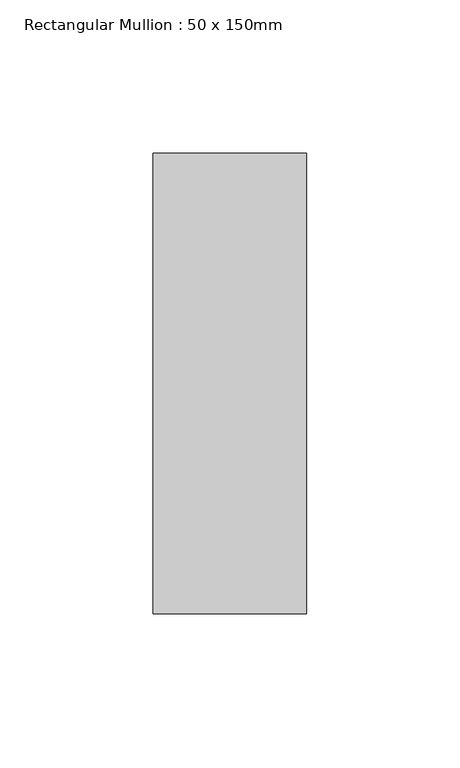
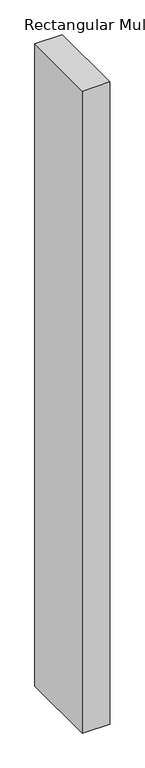
"""IFC4 building model written with IfcOpenShell, lengths in millimetres: member geometry, Rectangular Mullion : 50 x 150mm."""

from ifc_helpers import new_model, si_unit, frame, origin, place, context, project, spatial, polyline, outline, extrude, source, transform, mapped, element, save


def rectangular_mullion_50_x_150mm_31ac4966(model_context):
    return source(origin(), model_context, "Body", "SweptSolid", [
        extrude(outline(polyline([(0.0, 75.0), (0.0, -75.0), (-50.0, -75.0), (-50.0, 75.0), (0.0, 75.0)])), frame((0.0, 0.0, -1241.1082713), z_axis=(0.0, 0.0, 1.0), x_axis=(1.0, 0.0, 0.0)), (0.0, 0.0, 1.0), 1241.1082713),
    ])


if __name__ == "__main__":
    model = new_model("IFC4")
    model_context = context("Model", 3, world=origin())
    ifc_project = project(units=[si_unit("LENGTHUNIT", "METRE", prefix="MILLI")], contexts=[model_context])
    site = spatial("IfcSite", under=ifc_project)
    building = spatial("IfcBuilding", under=site)
    placement = place(None, origin())
    rectangular_mullion_50_x_150mm_shape = rectangular_mullion_50_x_150mm_31ac4966(model_context)
    element("IfcMember", 1, ObjectType="Rectangular Mullion : 50 x 150mm", at=placement, inside=building, context=model_context, shape_type="MappedRepresentation", body=[
        mapped(rectangular_mullion_50_x_150mm_shape, transform((0.0, 0.0, 0.0), x_axis=(1.0, 0.0, 0.0), y_axis=(0.0, 1.0, 0.0), z_axis=(0.0, 0.0, 1.0))),
    ])
    save(model, "model.ifc")

# Revit data of these elements
# Type "Rectangular Mullion : 50 x 150mm"
#   built-in parameter 1007304 = 0.492126 (stored number, unit not read)
#   built-in parameter 1007301 = 0.082021 (stored number, unit not read)
#   built-in parameter 1007300 = 0.082021 (stored number, unit not read)
# Element 1 (IfcMember, "Rectangular Mullion : 50 x 150mm")
#   Materials on its faces: "Aluminium"
# Materials
#   "Aluminium": class "Metal", colour RGB 247 247 247, transparency 0, Description = "Aluminium 6061", Cost = 0
